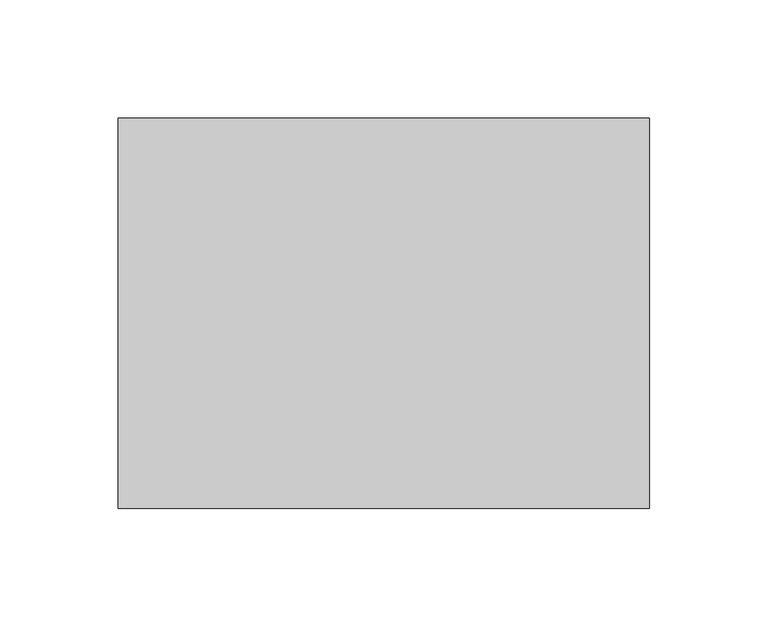
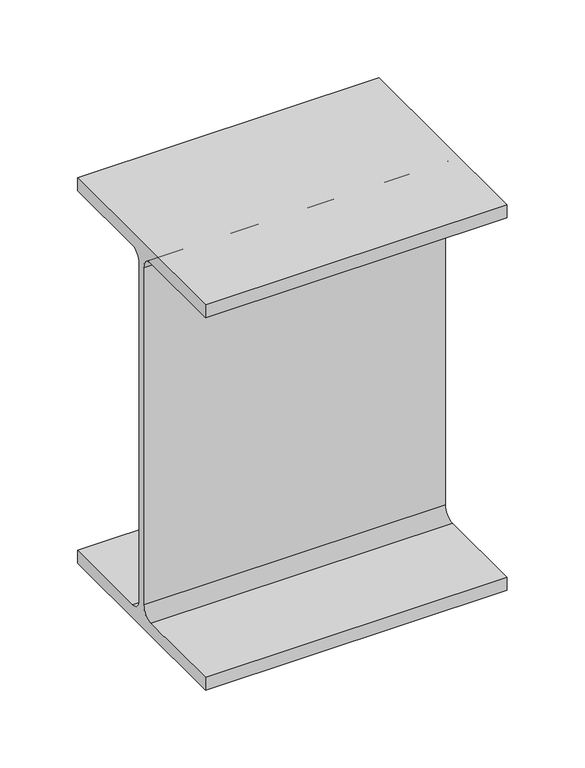
"""IFC4 building model written with IfcOpenShell, lengths in millimetres: beam geometry, Old_Steel Beam_H-KSD3502 : H_SB_ASB_H-300×150x6.5x9."""

from ifc_helpers import new_model, si_unit, point, frame, frame_2d, origin, place, context, project, spatial, polyline, circle_curve, trimmed, segment, composite_curve, outline, extrude, source, transform, mapped, element, save


def beam_59f34f2c(model_context):
    return source(origin(), model_context, "Body", "SweptSolid", [
        extrude(outline(composite_curve([segment(polyline([(82.5, -141.5), (82.5, -151.7), (-82.5, -151.7), (-82.5, -141.5), (-11.9, -141.5)]), True, "CONTINUOUS"), segment(trimmed(circle_curve(frame_2d((-11.9, -132.6)), 8.9), [point((-11.9, -141.5))], [point((-3.0, -132.6))], True, "CARTESIAN"), True, "CONTINUOUS"), segment(polyline([(-3.0, -132.6), (-3.0, 132.6)]), True, "CONTINUOUS"), segment(trimmed(circle_curve(frame_2d((-11.9, 132.6)), 8.9), [point((-3.0, 132.6))], [point((-11.9, 141.5))], True, "CARTESIAN"), True, "CONTINUOUS"), segment(polyline([(-11.9, 141.5), (-82.5, 141.5), (-82.5, 151.7), (82.5, 151.7), (82.5, 141.5), (11.9, 141.5)]), True, "CONTINUOUS"), segment(trimmed(circle_curve(frame_2d((11.9, 132.6)), 8.9), [point((11.9, 141.5))], [point((3.0, 132.6))], True, "CARTESIAN"), True, "CONTINUOUS"), segment(polyline([(3.0, 132.6), (3.0, -132.6)]), True, "CONTINUOUS"), segment(trimmed(circle_curve(frame_2d((11.9, -132.6)), 8.9), [point((3.0, -132.6))], [point((11.9, -141.5))], True, "CARTESIAN"), True, "CONTINUOUS"), segment(polyline([(11.9, -141.5), (82.5, -141.5)]), True, "CONTINUOUS")], self_intersect=False)), frame((-37.3, 0.0, 0.0), z_axis=(1.0, 0.0, 0.0), x_axis=(0.0, 1.0, 0.0)), (0.0, 0.0, 1.0), 224.5999994),
    ])


if __name__ == "__main__":
    model = new_model("IFC4")
    model_context = context("Model", 3, world=origin())
    ifc_project = project(units=[si_unit("LENGTHUNIT", "METRE", prefix="MILLI")], contexts=[model_context])
    site = spatial("IfcSite", under=ifc_project)
    building = spatial("IfcBuilding", under=site)
    placement = place(None, origin())
    beam_shape = beam_59f34f2c(model_context)
    element("IfcBeam", 1, ObjectType="Old_Steel Beam_H-KSD3502 : H_SB_ASB_H-300×150x6.5x9", at=placement, inside=building, context=model_context, shape_type="MappedRepresentation", body=[
        mapped(beam_shape, transform((0.0, 0.0, 0.0), x_axis=(1.0, 0.0, 0.0), y_axis=(0.0, 1.0, 0.0), z_axis=(0.0, 0.0, 1.0))),
    ])
    save(model, "model.ifc")

# Revit data of these elements
# Type "Old_Steel Beam_H-KSD3502 : H_SB_ASB_H-300×150x6.5x9"
#   Width = 15.0 cm
#   Web Thickness = 0.65 cm
#   Web Fillet = 1.3 cm
#   Warping Constant = 107174.0 cm⁶
#   Torsional Moment of Inertia = 9.9539 cm⁴
#   Torsional Modulus = 1.0 cm³
#   Section Area = 46.78 cm²
#   Plastic Modulus weak axis = 105.0 cm³
#   Plastic Modulus strong axis = 542.0 cm³
#   Perimeter = 1.17 m²/m
#   Nominal Weight = 36.70 kgf/m
#   Moment of Inertia weak axis = 508.00 cm⁴
#   Moment of Inertia strong axis = 7210.00 cm⁴
#   Height = 30.0 cm
#   Flange Thickness = 0.9 cm
#   Elastic Modulus weak axis = 67.7 cm³
#   Elastic Modulus strong axis = 481.0 cm³
#   Centroid Vertical = 15.0 cm
#   Centroid Horizontal = 7.5 cm
#   Length [instance default] = 1.5240 m
#   Structural Material [instance default] = Steel, 45-345
#   Assembly Code = ""
# Element 1 (IfcBeam, "Old_Steel Beam_H-KSD3502 : H_SB_ASB_H-300×150x6.5x9")
#   Structural Material = none
# Materials
#   "Steel, 45-345": class "Metal", colour RGB 189 187 185, transparency 0, Description = "Steel 345 MPa", Cost = 0
